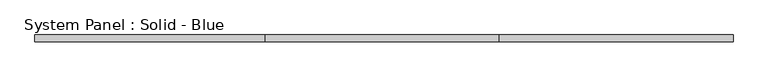
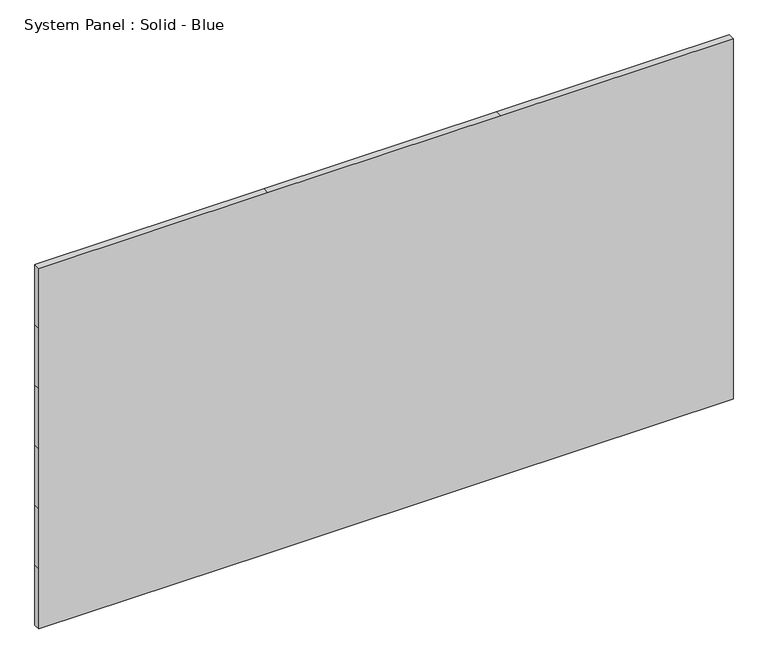
"""IFC4 building model written with IfcOpenShell, lengths in millimetres: plate geometry, System Panel : Solid - Blue."""

import ifcopenshell
import ifcopenshell.guid

model = None  # the IFC model being written
_history = None  # IfcOwnerHistory: only IFC2X3 demands one
_inside = {}  # id of a spatial element -> (the spatial element, [elements in it])
_under = {}  # id of a project, library or spatial element -> (it, [spatial elements below it])
_declared = {}  # id of a project -> (the project, [libraries it declares])
_typed = {}  # id of a type object -> (the type object, [elements of that type])
_made_of = {}  # id of a material, layer set ... -> (it, [elements and type objects made of it])


def new_model(schema):
    """Start an empty IFC model of exactly this schema.

    Asked for "IFC4X3", IfcOpenShell would pick the latest addendum, in which some entities
    have other attributes; the version numbers below select the first issue.
    IFC2X3 requires an IfcOwnerHistory on every rooted entity: one is made here for all.
    """
    global model, _history
    if schema == "IFC4X3":
        model = ifcopenshell.file(schema_version=(4, 3, 0, 0))
    else:
        model = ifcopenshell.file(schema=schema)
    _inside.clear()
    _under.clear()
    _declared.clear()
    _typed.clear()
    _made_of.clear()
    _history = None
    if model.schema == "IFC2X3":
        org = make("IfcOrganization", Name="unknown")
        user = make(
            "IfcPersonAndOrganization",
            ThePerson=make("IfcPerson", FamilyName="unknown"),
            TheOrganization=org,
        )
        app = make(
            "IfcApplication",
            ApplicationDeveloper=org,
            Version="unknown",
            ApplicationFullName="unknown",
            ApplicationIdentifier="unknown",
        )
        _history = make(
            "IfcOwnerHistory",
            OwningUser=user,
            OwningApplication=app,
            ChangeAction="ADDED",
            CreationDate=0,
        )
    return model


def make(cls, **values):
    """One entity of the class cls with the attributes given. An attribute that is None is left unset."""
    return model.create_entity(
        cls, **{name: value for name, value in values.items() if value is not None}
    )


def rooted(cls, **values):
    """An entity with a GlobalId (a new one), such as an element, a storey or a relation."""
    return make(cls, GlobalId=ifcopenshell.guid.new(), OwnerHistory=_history, **values)


def si_unit(unit_type, name, prefix=None):
    """IfcSIUnit, for example si_unit("LENGTHUNIT", "METRE", prefix="MILLI")."""
    return make("IfcSIUnit", UnitType=unit_type, Prefix=prefix, Name=name)


def assignment(units):
    """IfcUnitAssignment: the units of a project."""
    return None if units is None else make("IfcUnitAssignment", Units=units)


def point(xyz):
    """IfcCartesianPoint."""
    return None if xyz is None else make("IfcCartesianPoint", Coordinates=xyz)


def direction(xyz):
    """IfcDirection."""
    return None if xyz is None else make("IfcDirection", DirectionRatios=xyz)


def frame(location, z_axis=None, x_axis=None):
    """IfcAxis2Placement3D, a coordinate frame: its origin and axes. An axis left out is left unset."""
    return make(
        "IfcAxis2Placement3D",
        Location=point(location),
        Axis=direction(z_axis),
        RefDirection=direction(x_axis),
    )


def origin():
    """The frame at (0, 0, 0) with its axes left unset."""
    return frame((0.0, 0.0, 0.0))


def place(relative_to, where):
    """IfcLocalPlacement: puts the frame where relative to a parent placement (None: the world)."""
    return make(
        "IfcLocalPlacement", PlacementRelTo=relative_to, RelativePlacement=where
    )


def context(
    kind, dimensions, precision=None, world=None, true_north=None, identifier=None
):
    """IfcGeometricRepresentationContext, for example the 3D "Model" context."""
    return make(
        "IfcGeometricRepresentationContext",
        ContextIdentifier=identifier,
        ContextType=kind,
        CoordinateSpaceDimension=dimensions,
        Precision=precision,
        WorldCoordinateSystem=world,
        TrueNorth=true_north,
    )


def project(units=None, contexts=None):
    """IfcProject with its units and contexts."""
    return rooted(
        "IfcProject",
        Name="project",
        RepresentationContexts=contexts,
        UnitsInContext=assignment(units),
    )


def spatial(cls, under=None, at=None, **own):
    """A site, building, storey or space (cls), placed at a placement, below another one or the project."""
    s = rooted(cls, ObjectPlacement=at, **own)
    if under is not None:
        _under.setdefault(under.id(), (under, []))[1].append(s)
    return s


def polyline(points):
    """IfcPolyline through the points."""
    return make("IfcPolyline", Points=[point(p) for p in points])


def outline(outer, holes=None, kind="AREA"):
    """IfcArbitraryClosedProfileDef: a profile drawn as a closed curve; with holes, ...WithVoids."""
    if holes is None:
        return make("IfcArbitraryClosedProfileDef", ProfileType=kind, OuterCurve=outer)
    return make(
        "IfcArbitraryProfileDefWithVoids",
        ProfileType=kind,
        OuterCurve=outer,
        InnerCurves=holes,
    )


def extrude(swept, where, along, depth):
    """IfcExtrudedAreaSolid: the profile swept, set in the frame where, extruded along a direction by depth."""
    return make(
        "IfcExtrudedAreaSolid",
        SweptArea=swept,
        Position=where,
        ExtrudedDirection=direction(along),
        Depth=depth,
    )


def shape(context_of_items, identifier, shape_type, items):
    """IfcShapeRepresentation: the items that make up one representation, for example the "Body"."""
    return make(
        "IfcShapeRepresentation",
        ContextOfItems=context_of_items,
        RepresentationIdentifier=identifier,
        RepresentationType=shape_type,
        Items=items,
    )


def source(mapping_origin, context_of_items, identifier, shape_type, items):
    """IfcRepresentationMap: a shape defined once, which mapped items show again and again."""
    return make(
        "IfcRepresentationMap",
        MappingOrigin=mapping_origin,
        MappedRepresentation=shape(context_of_items, identifier, shape_type, items),
    )


def transform(
    local_origin,
    x_axis=None,
    y_axis=None,
    z_axis=None,
    scale=None,
    scale2=None,
    scale3=None,
    uniform=True,
):
    """IfcCartesianTransformationOperator3D, or its non-uniform kind. x_axis, y_axis, z_axis: its Axis1, 2, 3."""
    if uniform:
        return make(
            "IfcCartesianTransformationOperator3D",
            Axis1=direction(x_axis),
            Axis2=direction(y_axis),
            LocalOrigin=point(local_origin),
            Scale=scale,
            Axis3=direction(z_axis),
        )
    return make(
        "IfcCartesianTransformationOperator3DnonUniform",
        Axis1=direction(x_axis),
        Axis2=direction(y_axis),
        LocalOrigin=point(local_origin),
        Scale=scale,
        Axis3=direction(z_axis),
        Scale2=scale2,
        Scale3=scale3,
    )


def mapped(mapping_source, mapping_target):
    """IfcMappedItem: shows the shape of a source again, moved by a transform."""
    return make(
        "IfcMappedItem", MappingSource=mapping_source, MappingTarget=mapping_target
    )


def made_of(thing, what):
    """Note that an element or type object is made of a material, layer set ...; save() writes the relation."""
    if what is not None:
        _made_of.setdefault(what.id(), (what, []))[1].append(thing)
    return thing


def element(
    cls,
    number,
    at=None,
    inside=None,
    cuts=None,
    type_object=None,
    material=None,
    context=None,
    identifier="Body",
    shape_type=None,
    held_by="IfcProductDefinitionShape",
    body=None,
    shapes=None,
    **own,
):
    """One element of the class cls, such as IfcWall. Its Tag is "e" and its number.

    at: its placement. inside: the storey or other place that contains it. cuts: it is an
    opening in that element (IfcRelVoidsElement). A single representation is given by context,
    identifier, shape_type and body (its items); several are given by shapes. held_by: the class
    of the entity that holds the representations. save() writes the other relations.
    """
    e = rooted(cls, Tag="e%d" % number, ObjectPlacement=at, **own)
    if body is not None:
        shapes = [shape(context, identifier, shape_type, body)]
    if shapes is not None:
        e.Representation = make(held_by, Representations=shapes)
    if inside is not None:
        _inside.setdefault(inside.id(), (inside, []))[1].append(e)
    if cuts is not None:
        rooted(
            "IfcRelVoidsElement", RelatingBuildingElement=cuts, RelatedOpeningElement=e
        )
    if type_object is not None:
        _typed.setdefault(type_object.id(), (type_object, []))[1].append(e)
    return made_of(e, material)


def aggregate(whole, parts):
    """IfcRelAggregates: a whole, such as a stair, and the parts it consists of."""
    return rooted("IfcRelAggregates", RelatingObject=whole, RelatedObjects=parts)


def save(model, path):
    """Write the relations noted so far, then the file.

    IfcRelAggregates (storeys below a building ...), IfcRelContainedInSpatialStructure (elements
    in a storey), IfcRelDefinesByType, IfcRelAssociatesMaterial and IfcRelDeclares: one each for
    every whole, place, type object, material and project.
    """
    for whole, parts in _under.values():
        aggregate(whole, parts)
    for where, things in _inside.values():
        rooted(
            "IfcRelContainedInSpatialStructure",
            RelatedElements=things,
            RelatingStructure=where,
        )
    for kind, things in _typed.values():
        rooted("IfcRelDefinesByType", RelatedObjects=things, RelatingType=kind)
    for what, things in _made_of.values():
        rooted("IfcRelAssociatesMaterial", RelatedObjects=things, RelatingMaterial=what)
    for by, libraries in _declared.values():
        rooted("IfcRelDeclares", RelatingContext=by, RelatedDefinitions=libraries)
    model.write(path)


def system_panel_solid_blue_48cba8a6(model_context):
    return source(origin(), model_context, "Body", "SweptSolid", [
        extrude(outline(polyline([(0.0, -3329.305), (0.0, -1130.935), (0.0, 1099.185), (0.0, 3329.305), (609.6, 3329.305), (1219.2, 3329.305), (1828.8, 3329.305), (2438.4, 3329.305), (3048.0, 3329.305), (3657.6, 3329.305), (3657.6, 1099.185), (3657.6, -1130.935), (3657.6, -3329.305), (3048.0, -3329.305), (2438.4, -3329.305), (1828.8, -3329.305), (1219.2, -3329.305), (609.6, -3329.305), (0.0, -3329.305)])), frame((0.0, -19.05, 0.0), z_axis=(0.0, 1.0, 0.0), x_axis=(0.0, 0.0, 1.0)), (0.0, 0.0, 1.0), 63.5),
    ])


if __name__ == "__main__":
    model = new_model("IFC4")
    model_context = context("Model", 3, world=origin())
    ifc_project = project(units=[si_unit("LENGTHUNIT", "METRE", prefix="MILLI")], contexts=[model_context])
    site = spatial("IfcSite", under=ifc_project)
    building = spatial("IfcBuilding", under=site)
    placement = place(None, origin())
    system_panel_solid_blue_shape = system_panel_solid_blue_48cba8a6(model_context)
    element("IfcPlate", 1, ObjectType="System Panel : Solid - Blue", at=placement, inside=building, context=model_context, shape_type="MappedRepresentation", body=[
        mapped(system_panel_solid_blue_shape, transform((0.0, 0.0, 0.0), x_axis=(1.0, 0.0, 0.0), y_axis=(0.0, 1.0, 0.0), z_axis=(0.0, 0.0, 1.0))),
    ])
    save(model, "model.ifc")

# Revit data of these elements
# Project information
#   SR Document GUID = "95f8c40d-21e0-4786-882e-2c1e01a6cca9"
# Element 1 (IfcPlate, "System Panel : Solid - Blue")
#   Materials on its faces: "Blue Panel"
# Materials
#   "Blue Panel": class "Unassigned", colour RGB 0 0 160, transparency 0
